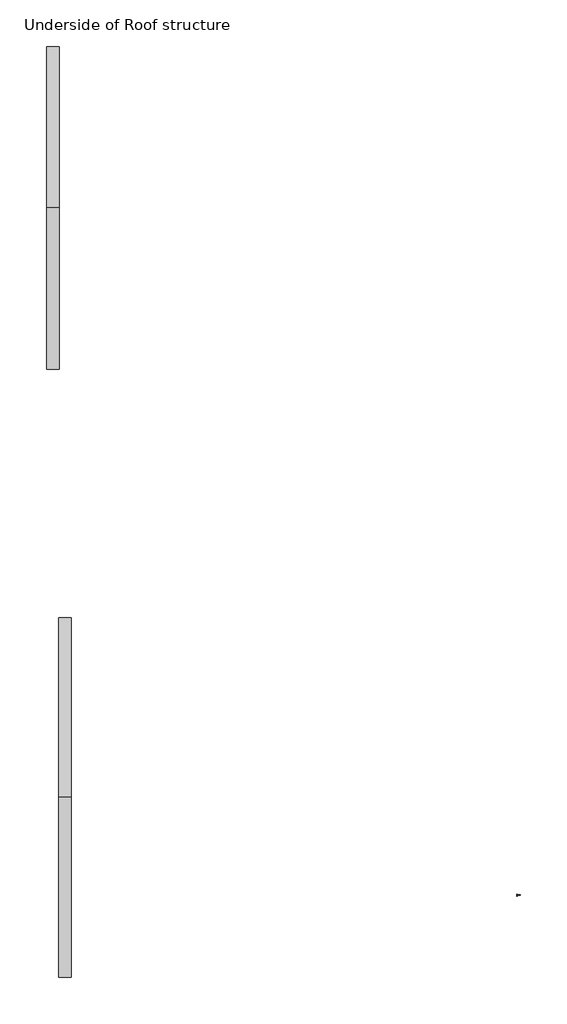
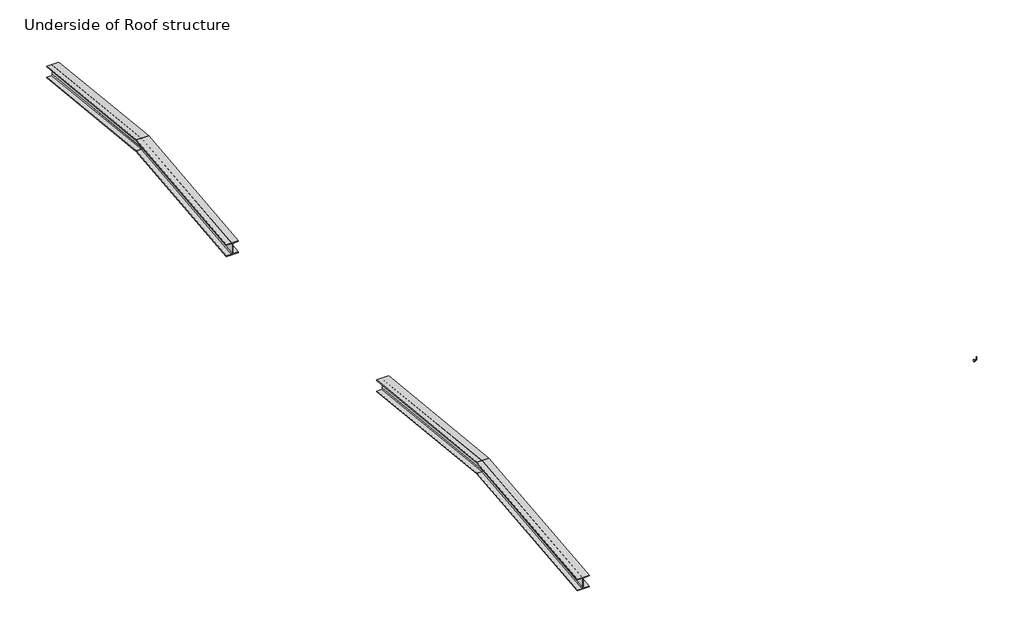
# One storey: 4 beams, 1 proxy.
"""IFC4 building model written with IfcOpenShell, lengths in millimetres."""

import ifcopenshell
import ifcopenshell.guid

model = None  # the IFC model being written
_history = None  # IfcOwnerHistory: only IFC2X3 demands one
_inside = {}  # id of a spatial element -> (the spatial element, [elements in it])
_under = {}  # id of a project, library or spatial element -> (it, [spatial elements below it])
_declared = {}  # id of a project -> (the project, [libraries it declares])
_typed = {}  # id of a type object -> (the type object, [elements of that type])
_made_of = {}  # id of a material, layer set ... -> (it, [elements and type objects made of it])


def new_model(schema):
    """Start an empty IFC model of exactly this schema.

    Asked for "IFC4X3", IfcOpenShell would pick the latest addendum, in which some entities
    have other attributes; the version numbers below select the first issue.
    IFC2X3 requires an IfcOwnerHistory on every rooted entity: one is made here for all.
    """
    global model, _history
    if schema == "IFC4X3":
        model = ifcopenshell.file(schema_version=(4, 3, 0, 0))
    else:
        model = ifcopenshell.file(schema=schema)
    _inside.clear()
    _under.clear()
    _declared.clear()
    _typed.clear()
    _made_of.clear()
    _history = None
    if model.schema == "IFC2X3":
        org = make("IfcOrganization", Name="unknown")
        user = make(
            "IfcPersonAndOrganization",
            ThePerson=make("IfcPerson", FamilyName="unknown"),
            TheOrganization=org,
        )
        app = make(
            "IfcApplication",
            ApplicationDeveloper=org,
            Version="unknown",
            ApplicationFullName="unknown",
            ApplicationIdentifier="unknown",
        )
        _history = make(
            "IfcOwnerHistory",
            OwningUser=user,
            OwningApplication=app,
            ChangeAction="ADDED",
            CreationDate=0,
        )
    return model


def make(cls, **values):
    """One entity of the class cls with the attributes given. An attribute that is None is left unset."""
    return model.create_entity(
        cls, **{name: value for name, value in values.items() if value is not None}
    )


def rooted(cls, **values):
    """An entity with a GlobalId (a new one), such as an element, a storey or a relation."""
    return make(cls, GlobalId=ifcopenshell.guid.new(), OwnerHistory=_history, **values)


def si_unit(unit_type, name, prefix=None):
    """IfcSIUnit, for example si_unit("LENGTHUNIT", "METRE", prefix="MILLI")."""
    return make("IfcSIUnit", UnitType=unit_type, Prefix=prefix, Name=name)


def assignment(units):
    """IfcUnitAssignment: the units of a project."""
    return None if units is None else make("IfcUnitAssignment", Units=units)


def point(xyz):
    """IfcCartesianPoint."""
    return None if xyz is None else make("IfcCartesianPoint", Coordinates=xyz)


def direction(xyz):
    """IfcDirection."""
    return None if xyz is None else make("IfcDirection", DirectionRatios=xyz)


def frame(location, z_axis=None, x_axis=None):
    """IfcAxis2Placement3D, a coordinate frame: its origin and axes. An axis left out is left unset."""
    return make(
        "IfcAxis2Placement3D",
        Location=point(location),
        Axis=direction(z_axis),
        RefDirection=direction(x_axis),
    )


def frame_2d(location, x_axis=None):
    """IfcAxis2Placement2D, a coordinate frame in the plane: its origin and x axis."""
    return make(
        "IfcAxis2Placement2D", Location=point(location), RefDirection=direction(x_axis)
    )


def origin():
    """The frame at (0, 0, 0) with its axes left unset."""
    return frame((0.0, 0.0, 0.0))


def origin_with_axes():
    """The frame at (0, 0, 0) with the z axis (0, 0, 1) and the x axis (1, 0, 0) written out."""
    return frame((0.0, 0.0, 0.0), z_axis=(0.0, 0.0, 1.0), x_axis=(1.0, 0.0, 0.0))


def place(relative_to, where):
    """IfcLocalPlacement: puts the frame where relative to a parent placement (None: the world)."""
    return make(
        "IfcLocalPlacement", PlacementRelTo=relative_to, RelativePlacement=where
    )


def context(
    kind, dimensions, precision=None, world=None, true_north=None, identifier=None
):
    """IfcGeometricRepresentationContext, for example the 3D "Model" context."""
    return make(
        "IfcGeometricRepresentationContext",
        ContextIdentifier=identifier,
        ContextType=kind,
        CoordinateSpaceDimension=dimensions,
        Precision=precision,
        WorldCoordinateSystem=world,
        TrueNorth=true_north,
    )


def project(units=None, contexts=None):
    """IfcProject with its units and contexts."""
    return rooted(
        "IfcProject",
        Name="project",
        RepresentationContexts=contexts,
        UnitsInContext=assignment(units),
    )


def spatial(cls, under=None, at=None, **own):
    """A site, building, storey or space (cls), placed at a placement, below another one or the project."""
    s = rooted(cls, ObjectPlacement=at, **own)
    if under is not None:
        _under.setdefault(under.id(), (under, []))[1].append(s)
    return s


def polyline(points):
    """IfcPolyline through the points."""
    return make("IfcPolyline", Points=[point(p) for p in points])


def circle_curve(where, radius):
    """IfcCircle in the frame where."""
    return make("IfcCircle", Position=where, Radius=radius)


def ellipse_curve(where, semi_axis1, semi_axis2):
    """IfcEllipse in the frame where."""
    return make(
        "IfcEllipse", Position=where, SemiAxis1=semi_axis1, SemiAxis2=semi_axis2
    )


def trimmed(basis, trim1, trim2, sense, master):
    """IfcTrimmedCurve: the piece of a basis curve between two trims."""
    return make(
        "IfcTrimmedCurve",
        BasisCurve=basis,
        Trim1=trim1,
        Trim2=trim2,
        SenseAgreement=sense,
        MasterRepresentation=master,
    )


def segment(curve, same_sense, transition):
    """IfcCompositeCurveSegment."""
    return make(
        "IfcCompositeCurveSegment",
        Transition=transition,
        SameSense=same_sense,
        ParentCurve=curve,
    )


def composite_curve(segments, self_intersect=None):
    """IfcCompositeCurve: segments joined end to end."""
    return make("IfcCompositeCurve", Segments=segments, SelfIntersect=self_intersect)


def outline(outer, holes=None, kind="AREA"):
    """IfcArbitraryClosedProfileDef: a profile drawn as a closed curve; with holes, ...WithVoids."""
    if holes is None:
        return make("IfcArbitraryClosedProfileDef", ProfileType=kind, OuterCurve=outer)
    return make(
        "IfcArbitraryProfileDefWithVoids",
        ProfileType=kind,
        OuterCurve=outer,
        InnerCurves=holes,
    )


def extrude(swept, where, along, depth):
    """IfcExtrudedAreaSolid: the profile swept, set in the frame where, extruded along a direction by depth."""
    return make(
        "IfcExtrudedAreaSolid",
        SweptArea=swept,
        Position=where,
        ExtrudedDirection=direction(along),
        Depth=depth,
    )


def shape(context_of_items, identifier, shape_type, items):
    """IfcShapeRepresentation: the items that make up one representation, for example the "Body"."""
    return make(
        "IfcShapeRepresentation",
        ContextOfItems=context_of_items,
        RepresentationIdentifier=identifier,
        RepresentationType=shape_type,
        Items=items,
    )


def source(mapping_origin, context_of_items, identifier, shape_type, items):
    """IfcRepresentationMap: a shape defined once, which mapped items show again and again."""
    return make(
        "IfcRepresentationMap",
        MappingOrigin=mapping_origin,
        MappedRepresentation=shape(context_of_items, identifier, shape_type, items),
    )


def transform(
    local_origin,
    x_axis=None,
    y_axis=None,
    z_axis=None,
    scale=None,
    scale2=None,
    scale3=None,
    uniform=True,
):
    """IfcCartesianTransformationOperator3D, or its non-uniform kind. x_axis, y_axis, z_axis: its Axis1, 2, 3."""
    if uniform:
        return make(
            "IfcCartesianTransformationOperator3D",
            Axis1=direction(x_axis),
            Axis2=direction(y_axis),
            LocalOrigin=point(local_origin),
            Scale=scale,
            Axis3=direction(z_axis),
        )
    return make(
        "IfcCartesianTransformationOperator3DnonUniform",
        Axis1=direction(x_axis),
        Axis2=direction(y_axis),
        LocalOrigin=point(local_origin),
        Scale=scale,
        Axis3=direction(z_axis),
        Scale2=scale2,
        Scale3=scale3,
    )


def mapped(mapping_source, mapping_target):
    """IfcMappedItem: shows the shape of a source again, moved by a transform."""
    return make(
        "IfcMappedItem", MappingSource=mapping_source, MappingTarget=mapping_target
    )


def made_of(thing, what):
    """Note that an element or type object is made of a material, layer set ...; save() writes the relation."""
    if what is not None:
        _made_of.setdefault(what.id(), (what, []))[1].append(thing)
    return thing


def element(
    cls,
    number,
    at=None,
    inside=None,
    cuts=None,
    type_object=None,
    material=None,
    context=None,
    identifier="Body",
    shape_type=None,
    held_by="IfcProductDefinitionShape",
    body=None,
    shapes=None,
    **own,
):
    """One element of the class cls, such as IfcWall. Its Tag is "e" and its number.

    at: its placement. inside: the storey or other place that contains it. cuts: it is an
    opening in that element (IfcRelVoidsElement). A single representation is given by context,
    identifier, shape_type and body (its items); several are given by shapes. held_by: the class
    of the entity that holds the representations. save() writes the other relations.
    """
    e = rooted(cls, Tag="e%d" % number, ObjectPlacement=at, **own)
    if body is not None:
        shapes = [shape(context, identifier, shape_type, body)]
    if shapes is not None:
        e.Representation = make(held_by, Representations=shapes)
    if inside is not None:
        _inside.setdefault(inside.id(), (inside, []))[1].append(e)
    if cuts is not None:
        rooted(
            "IfcRelVoidsElement", RelatingBuildingElement=cuts, RelatedOpeningElement=e
        )
    if type_object is not None:
        _typed.setdefault(type_object.id(), (type_object, []))[1].append(e)
    return made_of(e, material)


def aggregate(whole, parts):
    """IfcRelAggregates: a whole, such as a stair, and the parts it consists of."""
    return rooted("IfcRelAggregates", RelatingObject=whole, RelatedObjects=parts)


def save(model, path):
    """Write the relations noted so far, then the file.

    IfcRelAggregates (storeys below a building ...), IfcRelContainedInSpatialStructure (elements
    in a storey), IfcRelDefinesByType, IfcRelAssociatesMaterial and IfcRelDeclares: one each for
    every whole, place, type object, material and project.
    """
    for whole, parts in _under.values():
        aggregate(whole, parts)
    for where, things in _inside.values():
        rooted(
            "IfcRelContainedInSpatialStructure",
            RelatedElements=things,
            RelatingStructure=where,
        )
    for kind, things in _typed.values():
        rooted("IfcRelDefinesByType", RelatedObjects=things, RelatingType=kind)
    for what, things in _made_of.values():
        rooted("IfcRelAssociatesMaterial", RelatedObjects=things, RelatingMaterial=what)
    for by, libraries in _declared.values():
        rooted("IfcRelDeclares", RelatingContext=by, RelatedDefinitions=libraries)
    model.write(path)


def plane_surface(at):
    """IfcPlane: the flat surface through the origin of the frame at, square to its z axis."""
    return make("IfcPlane", Position=at)


def cylinder_surface(at, radius):
    """IfcCylindricalSurface: all points at the distance radius from the z axis of the frame at."""
    return make("IfcCylindricalSurface", Position=at, Radius=radius)


def revolved_surface(curve, axis_point, axis_direction):
    """IfcSurfaceOfRevolution: the curve turned about the line through axis_point along axis_direction."""
    return make(
        "IfcSurfaceOfRevolution",
        SweptCurve=make("IfcArbitraryOpenProfileDef", ProfileType="CURVE", Curve=curve),
        AxisPosition=make("IfcAxis1Placement", Location=point(axis_point), Axis=direction(axis_direction)),
    )


def advanced_brep(points, edges, surfaces, faces):
    """IfcAdvancedBrep: a solid bounded by faces that lie on surfaces and meet in shared edges.

    An edge is (start, end): straight between two places in points (the first is 0);
    or (start, end, curve); or (start, end, curve, False) where it runs against its curve.
    A face is (place in surfaces, loops), or (place, loops, False) where it looks against
    its surface's normal. A loop lists edges by number (the first is 1), with a minus sign
    where the edge is run from its end to its start. The first loop is the outer one.
    """
    corners = [point(p) for p in points]
    vertices = [make("IfcVertexPoint", VertexGeometry=c) for c in corners]
    made = []
    for start, end, *more in edges:
        made.append(
            make(
                "IfcEdgeCurve",
                EdgeStart=vertices[start],
                EdgeEnd=vertices[end],
                EdgeGeometry=more[0] if more else make("IfcPolyline", Points=[corners[start], corners[end]]),
                SameSense=more[1] if len(more) > 1 else True,
            )
        )
    hull = []
    for where, loops, *sense in faces:
        bounds = []
        for j, loop in enumerate(loops):
            ring = [make("IfcOrientedEdge", EdgeElement=made[abs(k) - 1], Orientation=k > 0) for k in loop]
            bounds.append(
                make(
                    "IfcFaceOuterBound" if j == 0 else "IfcFaceBound",
                    Bound=make("IfcEdgeLoop", EdgeList=ring),
                    Orientation=True,
                )
            )
        hull.append(make("IfcAdvancedFace", Bounds=bounds, FaceSurface=surfaces[where], SameSense=sense[0] if sense else True))
    return make("IfcAdvancedBrep", Outer=make("IfcClosedShell", CfsFaces=hull))


def support_metal_circular1_support_metal_circular_6fb01533(model_context):
    return source(origin(), model_context, "Body", "SolidModel", [
        advanced_brep(
        [(0.0, 63.5, -69.85), (0.0, 63.5, -82.55), (0.0, 12.7, -69.85), (0.0, 12.7, -82.55), (0.0, -6.35, -63.5), (0.0, 6.35, -63.5), (0.0, 6.35, 0.0), (0.0, -6.35, 0.0)],
        [
            (0, 1, circle_curve(frame((0.0, 63.5, -76.2), z_axis=(0.0, 1.0, 0.0), x_axis=(0.0, 0.0, -1.0)), 6.35)),
            (1, 0, circle_curve(frame((0.0, 63.5, -76.2), z_axis=(0.0, 1.0, 0.0), x_axis=(0.0, 0.0, -1.0)), 6.35)),
            (0, 2),
            (2, 3, circle_curve(frame((0.0, 12.7, -76.2), z_axis=(0.0, 1.0, 0.0), x_axis=(0.0, 0.0, -1.0)), 6.35)),
            (3, 1),
            (3, 2, circle_curve(frame((0.0, 12.7, -76.2), z_axis=(0.0, 1.0, 0.0), x_axis=(0.0, 0.0, -1.0)), 6.35)),
            (4, 3, circle_curve(frame((0.0, 12.7, -63.5), z_axis=(1.0, 0.0, 0.0), x_axis=(0.0, 0.0, -1.0)), 19.05)),
            (2, 5, circle_curve(frame((0.0, 12.7, -63.5), z_axis=(-1.0, 0.0, 0.0), x_axis=(0.0, 0.0, -1.0)), 6.35)),
            (5, 4, circle_curve(frame((0.0, 0.0, -63.5), z_axis=(0.0, 0.0, -1.0), x_axis=(0.0, -1.0, 0.0)), 6.35)),
            (4, 5, circle_curve(frame((0.0, 0.0, -63.5), z_axis=(0.0, 0.0, -1.0), x_axis=(0.0, -1.0, 0.0)), 6.35)),
            (6, 7, circle_curve(frame((0.0, 0.0, 0.0), z_axis=(0.0, 0.0, 1.0), x_axis=(0.0, -1.0, 0.0)), 6.35)),
            (7, 6, circle_curve(frame((0.0, 0.0, 0.0), z_axis=(0.0, 0.0, 1.0), x_axis=(0.0, -1.0, 0.0)), 6.35)),
            (5, 6),
            (7, 4),
        ],
        [
            plane_surface(frame((0.0, 63.5, -76.2), z_axis=(0.0, 1.0, 0.0), x_axis=(1.0, 0.0, 0.0))),
            cylinder_surface(frame((0.0, 63.5, -76.2), z_axis=(0.0, 1.0, 0.0), x_axis=(0.0, 0.0, -1.0)), 6.35),
            revolved_surface(trimmed(ellipse_curve(frame((0.0, 12.7, -76.2), z_axis=(0.0, 1.0, 0.0), x_axis=(0.0, 0.0, -1.0)), 6.35, 6.35), [point((0.0, 12.7, -69.85))], [point((0.0, 12.7, -82.55))], True, "CARTESIAN"), (0.0, 12.7, -63.5), (-1.0, 0.0, 0.0)),
            revolved_surface(trimmed(ellipse_curve(frame((0.0, 12.7, -76.2), z_axis=(0.0, 1.0, 0.0), x_axis=(0.0, 0.0, -1.0)), 6.35, 6.35), [point((0.0, 12.7, -82.55))], [point((0.0, 12.7, -69.85))], True, "CARTESIAN"), (0.0, 12.7, -63.5), (-1.0, 0.0, 0.0)),
            plane_surface(origin_with_axes()),
            cylinder_surface(frame((0.0, 0.0, -63.5), z_axis=(0.0, 0.0, -1.0), x_axis=(0.0, -1.0, 0.0)), 6.35),
        ],
        [
            (0, [[1, 2]]),
            (1, [[-1, 3, 4, 5]]),
            (1, [[-2, -5, 6, -3]]),
            (2, [[7, -4, 8, 9]]),
            (3, [[-8, -6, -7, 10]]),
            (4, [[11, 12]]),
            (5, [[-9, 13, -12, 14]]),
            (5, [[-10, -14, -11, -13]]),
        ],
    ),
        extrude(outline(composite_curve([segment(trimmed(circle_curve(frame_2d((-76.2, 0.0)), 25.4), [point((-76.2, -25.4))], [point((-76.2, 25.4))], False, "CARTESIAN"), True, "CONTINUOUS"), segment(trimmed(circle_curve(frame_2d((-76.2, 0.0)), 25.4), [point((-76.2, 25.4))], [point((-76.2, -25.4))], False, "CARTESIAN"), True, "CONTINUOUS")], self_intersect=False)), frame((0.0, 63.5, 0.0), z_axis=(0.0, 1.0, 0.0), x_axis=(0.0, 0.0, 1.0)), (0.0, 0.0, 1.0), 12.7),
    ])


model = new_model("IFC4")

# Units and contexts
model_context = context("Model", 3, world=origin())
ifc_project = project(units=[si_unit("LENGTHUNIT", "METRE", prefix="MILLI")], contexts=[model_context])

# Site, building, storey
site = spatial("IfcSite", under=ifc_project)
building = spatial("IfcBuilding", under=site)
storey = spatial("IfcBuildingStorey", under=building, Name="Underside of Roof structure", Elevation=34036.0)

# Beams
placement = place(None, origin())
element("IfcBeam", 1, ObjectType="W-Wide Flange : W12X79", at=placement, inside=storey, context=model_context, shape_type="AdvancedBrep", body=[
    advanced_brep(
    [(-21755.4154607, 20844.8695005, 33191.9562864), (-21755.4154607, 16882.4695005, 33611.0562864), (-21630.3204607, 16882.4695005, 33611.0562864), (-21630.3204607, 20844.8695005, 33191.9562864), (-21755.4154607, 20844.8695005, 33173.1831506), (-21755.4154607, 16882.4695005, 33592.2831506), (-21448.0754607, 16882.4695005, 33592.2831506), (-21448.0754607, 16882.4695005, 33611.0562864), (-21573.1704607, 16882.4695005, 33611.0562864), (-21595.7764607, 16882.4695005, 33633.7883829), (-21595.7764607, 16882.4695005, 33867.4947677), (-21573.1704607, 16882.4695005, 33890.2268642), (-21448.0754607, 16882.4695005, 33890.2268642), (-21448.0754607, 16882.4695005, 33909.0), (-21755.4154607, 16882.4695005, 33909.0), (-21755.4154607, 16882.4695005, 33890.2268642), (-21630.3204607, 16882.4695005, 33890.2268642), (-21607.7144607, 16882.4695005, 33867.4947677), (-21607.7144607, 16882.4695005, 33633.7883829), (-21607.7144607, 20844.8695005, 33214.6883829), (-21607.7144607, 20844.8695005, 33448.3947677), (-21630.3204607, 20844.8695005, 33471.1268642), (-21755.4154607, 20844.8695005, 33471.1268642), (-21755.4154607, 20844.8695005, 33489.9), (-21448.0754607, 20844.8695005, 33489.9), (-21448.0754607, 20844.8695005, 33471.1268642), (-21573.1704607, 20844.8695005, 33471.1268642), (-21595.7764607, 20844.8695005, 33448.3947677), (-21595.7764607, 20844.8695005, 33214.6883829), (-21573.1704607, 20844.8695005, 33191.9562864), (-21448.0754607, 20844.8695005, 33191.9562864), (-21448.0754607, 20844.8695005, 33173.1831506)],
    [
        (0, 1),
        (1, 2),
        (2, 3),
        (3, 0),
        (4, 5),
        (5, 1),
        (0, 4),
        (5, 6),
        (6, 7),
        (7, 8),
        (8, 9, ellipse_curve(frame((-21573.1704607, 16882.4695005, 33633.7883829), z_axis=(0.0, 1.0, 0.0), x_axis=(0.0, 0.0, 0.9999999999999999)), 22.7320964, 22.606)),
        (9, 10),
        (10, 11, ellipse_curve(frame((-21573.1704607, 16882.4695005, 33867.4947677), z_axis=(0.0, 1.0, 0.0), x_axis=(0.0, 0.0, 0.9999999999999999)), 22.7320964, 22.606)),
        (11, 12),
        (12, 13),
        (13, 14),
        (14, 15),
        (15, 16),
        (16, 17, ellipse_curve(frame((-21630.3204607, 16882.4695005, 33867.4947677), z_axis=(0.0, 1.0, 0.0), x_axis=(0.0, 0.0, 0.9999999999999999)), 22.7320964, 22.606)),
        (17, 18),
        (18, 2, ellipse_curve(frame((-21630.3204607, 16882.4695005, 33633.7883829), z_axis=(0.0, 1.0, 0.0), x_axis=(0.0, 0.0, 0.9999999999999999)), 22.7320964, 22.606)),
        (18, 19),
        (19, 3, ellipse_curve(frame((-21630.3204607, 20844.8695005, 33214.6883829), z_axis=(0.0, 1.0, 0.0), x_axis=(0.0, 0.0, 0.9999999999999999)), 22.7320964, 22.606)),
        (17, 20),
        (20, 19),
        (16, 21),
        (21, 20, ellipse_curve(frame((-21630.3204607, 20844.8695005, 33448.3947677), z_axis=(0.0, 1.0, 0.0), x_axis=(0.0, 0.0, 0.9999999999999999)), 22.7320964, 22.606)),
        (15, 22),
        (22, 21),
        (14, 23),
        (23, 22),
        (13, 24),
        (24, 23),
        (12, 25),
        (25, 24),
        (11, 26),
        (26, 25),
        (10, 27),
        (27, 26, ellipse_curve(frame((-21573.1704607, 20844.8695005, 33448.3947677), z_axis=(0.0, 1.0, 0.0), x_axis=(0.0, 0.0, 0.9999999999999999)), 22.7320964, 22.606)),
        (9, 28),
        (28, 27),
        (8, 29),
        (29, 28, ellipse_curve(frame((-21573.1704607, 20844.8695005, 33214.6883829), z_axis=(0.0, 1.0, 0.0), x_axis=(0.0, 0.0, 0.9999999999999999)), 22.7320964, 22.606)),
        (7, 30),
        (30, 29),
        (6, 31),
        (31, 30),
        (4, 31),
    ],
    [
        plane_surface(frame((-21692.8679607, 20969.2190095, 33178.8039345), z_axis=(0.0, 0.10518252182083103, 0.9944529335787644), x_axis=(1.0, 0.0, 0.0))),
        plane_surface(frame((-21755.4154607, 20968.2371832, 33169.5212136), z_axis=(-1.0, 0.0, 0.0), x_axis=(0.0, 0.10518252182083183, 0.9944529335787644))),
        plane_surface(frame((-21601.7454607, 16882.4695005, 33592.2831506), z_axis=(0.0, -1.0, 0.0), x_axis=(0.0, 0.0, 1.0))),
        revolved_surface(polyline([(-21607.7144607, 16880.091744411304, 33634.03987627958), (-21607.7144607, 20847.247256588096, 33214.43688941473)]), (-21630.3204607, 20971.5967656, 33201.2845375), (0.0, -0.9944529335787643, 0.10518252182083102)),
        plane_surface(frame((-21607.7144607, 20983.8195005, 33316.8449407), z_axis=(-1.0, 0.0, 0.0), x_axis=(0.0, 0.10518252182083183, 0.9944529335787644))),
        revolved_surface(polyline([(-21630.3204607, 16882.46950049405, 33890.226864143755), (-21630.3204607, 20849.625012670844, 33470.6238772789)]), (-21630.3204607, 20996.0422355, 33432.4053438), (0.0, -0.9944529335787643, 0.10518252182083102)),
        plane_surface(frame((-21692.8679607, 20998.4199915, 33454.8859468), z_axis=(0.0, -0.10518252182083103, -0.9944529335787644), x_axis=(-1.0, 0.0, 0.0))),
        plane_surface(frame((-21755.4154607, 20999.4018178, 33464.1686678), z_axis=(-1.0, 0.0, 0.0), x_axis=(0.0, 0.10518252182083183, 0.9944529335787644))),
        plane_surface(frame((-21601.7454607, 21000.383644, 33473.4513887), z_axis=(0.0, 0.10518252182083103, 0.9944529335787644), x_axis=(1.0, 0.0, 0.0))),
        plane_surface(frame((-21448.0754607, 20999.4018178, 33464.1686678), z_axis=(1.0, 0.0, 0.0), x_axis=(0.0, -0.10518252182083183, -0.9944529335787644))),
        plane_surface(frame((-21510.6229607, 20998.4199915, 33454.8859468), z_axis=(0.0, -0.10518252182083103, -0.9944529335787644), x_axis=(-1.0, 0.0, 0.0))),
        revolved_surface(polyline([(-21595.7764607, 16880.09174440577, 33867.74626112727), (-21595.7764607, 20847.247256582563, 33448.14327426242)]), (-21573.1704607, 20996.0422355, 33432.4053438), (0.0, -0.9944529335787643, 0.10518252182083102)),
        plane_surface(frame((-21595.7764607, 20983.8195005, 33316.8449407), z_axis=(1.0, 0.0, 0.0), x_axis=(0.0, -0.10518252182083183, -0.9944529335787644))),
        revolved_surface(polyline([(-21573.1704607, 16877.713988323023, 33611.5592732631), (-21573.1704607, 20844.869500499815, 33191.95628639824)]), (-21573.1704607, 20971.5967656, 33201.2845375), (0.0, -0.9944529335787643, 0.10518252182083102)),
        plane_surface(frame((-21510.6229607, 20969.2190095, 33178.8039345), z_axis=(0.0, 0.10518252182083103, 0.9944529335787644), x_axis=(1.0, 0.0, 0.0))),
        plane_surface(frame((-21448.0754607, 20968.2371832, 33169.5212136), z_axis=(1.0, 0.0, 0.0), x_axis=(0.0, -0.10518252182083183, -0.9944529335787644))),
        plane_surface(frame((-21601.7454607, 20967.255357, 33160.2384927), z_axis=(0.0, -0.10518252182083103, -0.9944529335787644), x_axis=(-1.0, 0.0, 0.0))),
        plane_surface(frame((-23272.9998994, 20844.8695005, 33801.3683204), z_axis=(0.0, 1.0, 0.0), x_axis=(0.0, 0.0, 1.0))),
    ],
    [
        (0, [[1, 2, 3, 4]]),
        (1, [[5, 6, -1, 7]]),
        (2, [[-6, 8, 9, 10, 11, 12, 13, 14, 15, 16, 17, 18, 19, 20, 21, -2]]),
        (3, [[-3, -21, 22, 23]]),
        (4, [[-22, -20, 24, 25]]),
        (5, [[-24, -19, 26, 27]]),
        (6, [[-26, -18, 28, 29]]),
        (7, [[-28, -17, 30, 31]]),
        (8, [[-30, -16, 32, 33]]),
        (9, [[-32, -15, 34, 35]]),
        (10, [[-34, -14, 36, 37]]),
        (11, [[-36, -13, 38, 39]]),
        (12, [[-38, -12, 40, 41]]),
        (13, [[-40, -11, 42, 43]]),
        (14, [[-42, -10, 44, 45]]),
        (15, [[-44, -9, 46, 47]]),
        (16, [[-46, -8, -5, 48]]),
        (17, [[-4, -23, -25, -27, -29, -31, -33, -35, -37, -39, -41, -43, -45, -47, -48, -7]]),
    ],
),
])
element("IfcBeam", 2, ObjectType="W-Wide Flange : W12X79", at=placement, inside=storey, context=model_context, shape_type="AdvancedBrep", body=[
    advanced_brep(
    [(-21607.7144607, 12920.0695005, 33214.6883829), (-21607.7144607, 16882.4695005, 33633.7883829), (-21630.3204607, 16882.4695005, 33611.0562864), (-21630.3204607, 12920.0695005, 33191.9562864), (-21755.4154607, 16882.4695005, 33611.0562864), (-21755.4154607, 12920.0695005, 33191.9562864), (-21607.7144607, 16882.4695005, 33867.4947677), (-21630.3204607, 16882.4695005, 33890.2268642), (-21755.4154607, 16882.4695005, 33890.2268642), (-21755.4154607, 16882.4695005, 33909.0), (-21448.0754607, 16882.4695005, 33909.0), (-21448.0754607, 16882.4695005, 33890.2268642), (-21573.1704607, 16882.4695005, 33890.2268642), (-21595.7764607, 16882.4695005, 33867.4947677), (-21595.7764607, 16882.4695005, 33633.7883829), (-21573.1704607, 16882.4695005, 33611.0562864), (-21448.0754607, 16882.4695005, 33611.0562864), (-21448.0754607, 16882.4695005, 33592.2831506), (-21755.4154607, 16882.4695005, 33592.2831506), (-21755.4154607, 12920.0695005, 33173.1831506), (-21607.7144607, 12920.0695005, 33448.3947677), (-21630.3204607, 12920.0695005, 33471.1268642), (-21755.4154607, 12920.0695005, 33471.1268642), (-21755.4154607, 12920.0695005, 33489.9), (-21448.0754607, 12920.0695005, 33489.9), (-21448.0754607, 12920.0695005, 33471.1268642), (-21573.1704607, 12920.0695005, 33471.1268642), (-21595.7764607, 12920.0695005, 33448.3947677), (-21595.7764607, 12920.0695005, 33214.6883829), (-21573.1704607, 12920.0695005, 33191.9562864), (-21448.0754607, 12920.0695005, 33191.9562864), (-21448.0754607, 12920.0695005, 33173.1831506)],
    [
        (0, 1),
        (1, 2, ellipse_curve(frame((-21630.3204607, 16882.4695005, 33633.7883829), z_axis=(0.0, 1.0, 0.0), x_axis=(0.0, 0.0, 1.0)), 22.7320964, 22.606)),
        (2, 3),
        (3, 0, ellipse_curve(frame((-21630.3204607, 12920.0695005, 33214.6883829), z_axis=(0.0, -1.0, 0.0), x_axis=(0.0, 0.0, 1.0)), 22.7320964, 22.606)),
        (2, 4),
        (4, 5),
        (5, 3),
        (1, 6),
        (6, 7, ellipse_curve(frame((-21630.3204607, 16882.4695005, 33867.4947677), z_axis=(0.0, -1.0, 0.0), x_axis=(0.0, 0.0, 1.0)), 22.7320964, 22.606)),
        (7, 8),
        (8, 9),
        (9, 10),
        (10, 11),
        (11, 12),
        (12, 13, ellipse_curve(frame((-21573.1704607, 16882.4695005, 33867.4947677), z_axis=(0.0, -1.0, 0.0), x_axis=(0.0, 0.0, 1.0)), 22.7320964, 22.606)),
        (13, 14),
        (14, 15, ellipse_curve(frame((-21573.1704607, 16882.4695005, 33633.7883829), z_axis=(0.0, -1.0, 0.0), x_axis=(0.0, 0.0, 1.0)), 22.7320964, 22.606)),
        (15, 16),
        (16, 17),
        (17, 18),
        (18, 4),
        (18, 19),
        (19, 5),
        (20, 6),
        (0, 20),
        (21, 7),
        (20, 21, ellipse_curve(frame((-21630.3204607, 12920.0695005, 33448.3947677), z_axis=(0.0, -1.0, 0.0), x_axis=(0.0, 0.0, 1.0)), 22.7320964, 22.606)),
        (22, 8),
        (21, 22),
        (23, 9),
        (22, 23),
        (24, 10),
        (23, 24),
        (25, 11),
        (24, 25),
        (26, 12),
        (25, 26),
        (27, 13),
        (26, 27, ellipse_curve(frame((-21573.1704607, 12920.0695005, 33448.3947677), z_axis=(0.0, -1.0, 0.0), x_axis=(0.0, 0.0, 1.0)), 22.7320964, 22.606)),
        (28, 14),
        (27, 28),
        (29, 15),
        (28, 29, ellipse_curve(frame((-21573.1704607, 12920.0695005, 33214.6883829), z_axis=(0.0, -1.0, 0.0), x_axis=(0.0, 0.0, 1.0)), 22.7320964, 22.606)),
        (30, 16),
        (29, 30),
        (31, 17),
        (30, 31),
        (31, 19),
    ],
    [
        revolved_surface(polyline([(-21607.7144607, 16884.847256589805, 33634.03987626912), (-21607.7144607, 12917.69174441301, 33214.436889404264)]), (-21630.3204607, 12793.3422355, 33201.2845375), (0.0, 0.9944529335787644, 0.10518252182083103)),
        plane_surface(frame((-21692.8679607, 12795.7199915, 33178.8039345), z_axis=(0.0, -0.10518252182083103, 0.9944529335787644), x_axis=(1.0, 0.0, 0.0))),
        plane_surface(frame((-21601.7454607, 16882.4695005, 33592.2831506), z_axis=(0.0, 1.0, 0.0), x_axis=(0.0, 0.0, -1.0))),
        plane_surface(frame((-21755.4154607, 12796.7018178, 33169.5212136), z_axis=(-1.0, 0.0, 0.0), x_axis=(0.0, -0.10518252182083185, 0.9944529335787644))),
        plane_surface(frame((-21607.7144607, 12781.1195005, 33316.8449407), z_axis=(-1.0, 0.0, 0.0), x_axis=(0.0, -0.10518252182083185, 0.9944529335787644))),
        revolved_surface(polyline([(-21630.3204607, 16882.469500507057, 33890.2268641333), (-21630.3204607, 12915.313988330263, 33470.623877268445)]), (-21630.3204607, 12768.8967656, 33432.4053438), (0.0, 0.9944529335787644, 0.10518252182083103)),
        plane_surface(frame((-21692.8679607, 12766.5190095, 33454.8859468), z_axis=(0.0, 0.10518252182083103, -0.9944529335787644), x_axis=(-1.0, 0.0, 0.0))),
        plane_surface(frame((-21755.4154607, 12765.5371832, 33464.1686678), z_axis=(-1.0, 0.0, 0.0), x_axis=(0.0, -0.10518252182083185, 0.9944529335787644))),
        plane_surface(frame((-21601.7454607, 12764.555357, 33473.4513887), z_axis=(0.0, -0.10518252182083103, 0.9944529335787644), x_axis=(1.0, 0.0, 0.0))),
        plane_surface(frame((-21448.0754607, 12765.5371832, 33464.1686678), z_axis=(1.0, 0.0, 0.0), x_axis=(0.0, 0.10518252182083185, -0.9944529335787644))),
        plane_surface(frame((-21510.6229607, 12766.5190095, 33454.8859468), z_axis=(0.0, 0.10518252182083103, -0.9944529335787644), x_axis=(-1.0, 0.0, 0.0))),
        revolved_surface(polyline([(-21595.7764607, 16884.847256595338, 33867.746261116816), (-21595.7764607, 12917.691744418544, 33448.14327425196)]), (-21573.1704607, 12768.8967656, 33432.4053438), (0.0, 0.9944529335787644, 0.10518252182083103)),
        plane_surface(frame((-21595.7764607, 12781.1195005, 33316.8449407), z_axis=(1.0, 0.0, 0.0), x_axis=(0.0, 0.10518252182083185, -0.9944529335787644))),
        revolved_surface(polyline([(-21573.1704607, 16887.225012678085, 33611.559273252635), (-21573.1704607, 12920.069500501291, 33191.95628638778)]), (-21573.1704607, 12793.3422355, 33201.2845375), (0.0, 0.9944529335787644, 0.10518252182083103)),
        plane_surface(frame((-21510.6229607, 12795.7199915, 33178.8039345), z_axis=(0.0, -0.10518252182083103, 0.9944529335787644), x_axis=(1.0, 0.0, 0.0))),
        plane_surface(frame((-21448.0754607, 12796.7018178, 33169.5212136), z_axis=(1.0, 0.0, 0.0), x_axis=(0.0, 0.10518252182083185, -0.9944529335787644))),
        plane_surface(frame((-21601.7454607, 12797.683644, 33160.2384927), z_axis=(0.0, 0.10518252182083103, -0.9944529335787644), x_axis=(-1.0, 0.0, 0.0))),
        plane_surface(frame((-23272.9998994, 12920.0695005, 33801.3683204), z_axis=(0.0, -1.0, 0.0), x_axis=(0.0, 0.0, 1.0))),
    ],
    [
        (0, [[1, 2, 3, 4]]),
        (1, [[-3, 5, 6, 7]]),
        (2, [[-5, -2, 8, 9, 10, 11, 12, 13, 14, 15, 16, 17, 18, 19, 20, 21]]),
        (3, [[-6, -21, 22, 23]]),
        (4, [[24, -8, -1, 25]]),
        (5, [[26, -9, -24, 27]]),
        (6, [[28, -10, -26, 29]]),
        (7, [[30, -11, -28, 31]]),
        (8, [[32, -12, -30, 33]]),
        (9, [[34, -13, -32, 35]]),
        (10, [[36, -14, -34, 37]]),
        (11, [[38, -15, -36, 39]]),
        (12, [[40, -16, -38, 41]]),
        (13, [[42, -17, -40, 43]]),
        (14, [[44, -18, -42, 45]]),
        (15, [[46, -19, -44, 47]]),
        (16, [[-22, -20, -46, 48]]),
        (17, [[-7, -23, -48, -47, -45, -43, -41, -39, -37, -35, -33, -31, -29, -27, -25, -4]]),
    ],
),
])
element("IfcBeam", 3, ObjectType="W-Wide Flange : W12X79", at=placement, inside=storey, context=model_context, shape_type="AdvancedBrep", body=[
    advanced_brep(
    [(-21450.6154607, 6824.0695005, 33143.5985941), (-21450.6154607, 2404.4695005, 33611.0562864), (-21325.5204607, 2404.4695005, 33611.0562864), (-21325.5204607, 6824.0695005, 33143.5985941), (-21450.6154607, 6824.0695005, 33124.8254583), (-21450.6154607, 2404.4695005, 33592.2831506), (-21143.2754607, 2404.4695005, 33592.2831506), (-21143.2754607, 2404.4695005, 33611.0562864), (-21268.3704607, 2404.4695005, 33611.0562864), (-21290.9764607, 2404.4695005, 33633.7883829), (-21290.9764607, 2404.4695005, 33867.4947677), (-21268.3704607, 2404.4695005, 33890.2268642), (-21143.2754607, 2404.4695005, 33890.2268642), (-21143.2754607, 2404.4695005, 33909.0), (-21450.6154607, 2404.4695005, 33909.0), (-21450.6154607, 2404.4695005, 33890.2268642), (-21325.5204607, 2404.4695005, 33890.2268642), (-21302.9144607, 2404.4695005, 33867.4947677), (-21302.9144607, 2404.4695005, 33633.7883829), (-21302.9144607, 6824.0695005, 33166.3306906), (-21302.9144607, 6824.0695005, 33400.0370754), (-21325.5204607, 6824.0695005, 33422.7691719), (-21450.6154607, 6824.0695005, 33422.7691719), (-21450.6154607, 6824.0695005, 33441.5423077), (-21143.2754607, 6824.0695005, 33441.5423077), (-21143.2754607, 6824.0695005, 33422.7691719), (-21268.3704607, 6824.0695005, 33422.7691719), (-21290.9764607, 6824.0695005, 33400.0370754), (-21290.9764607, 6824.0695005, 33166.3306906), (-21268.3704607, 6824.0695005, 33143.5985941), (-21143.2754607, 6824.0695005, 33143.5985941), (-21143.2754607, 6824.0695005, 33124.8254583)],
    [
        (0, 1),
        (1, 2),
        (2, 3),
        (3, 0),
        (4, 5),
        (5, 1),
        (0, 4),
        (5, 6),
        (6, 7),
        (7, 8),
        (8, 9, ellipse_curve(frame((-21268.3704607, 2404.4695005, 33633.7883829), z_axis=(0.0, 1.0, 0.0), x_axis=(0.0, 0.0, 0.9999999999999999)), 22.7320964, 22.606)),
        (9, 10),
        (10, 11, ellipse_curve(frame((-21268.3704607, 2404.4695005, 33867.4947677), z_axis=(0.0, 1.0, 0.0), x_axis=(0.0, 0.0, 0.9999999999999999)), 22.7320964, 22.606)),
        (11, 12),
        (12, 13),
        (13, 14),
        (14, 15),
        (15, 16),
        (16, 17, ellipse_curve(frame((-21325.5204607, 2404.4695005, 33867.4947677), z_axis=(0.0, 1.0, 0.0), x_axis=(0.0, 0.0, 0.9999999999999999)), 22.7320964, 22.606)),
        (17, 18),
        (18, 2, ellipse_curve(frame((-21325.5204607, 2404.4695005, 33633.7883829), z_axis=(0.0, 1.0, 0.0), x_axis=(0.0, 0.0, 0.9999999999999999)), 22.7320964, 22.606)),
        (18, 19),
        (19, 3, ellipse_curve(frame((-21325.5204607, 6824.0695005, 33166.3306906), z_axis=(0.0, 1.0, 0.0), x_axis=(0.0, 0.0, 0.9999999999999999)), 22.7320964, 22.606)),
        (17, 20),
        (20, 19),
        (16, 21),
        (21, 20, ellipse_curve(frame((-21325.5204607, 6824.0695005, 33400.0370754), z_axis=(0.0, 1.0, 0.0), x_axis=(0.0, 0.0, 0.9999999999999999)), 22.7320964, 22.606)),
        (15, 22),
        (22, 21),
        (14, 23),
        (23, 22),
        (13, 24),
        (24, 23),
        (12, 25),
        (25, 24),
        (11, 26),
        (26, 25),
        (10, 27),
        (27, 26, ellipse_curve(frame((-21268.3704607, 6824.0695005, 33400.0370754), z_axis=(0.0, 1.0, 0.0), x_axis=(0.0, 0.0, 0.9999999999999999)), 22.7320964, 22.606)),
        (9, 28),
        (28, 27),
        (8, 29),
        (29, 28, ellipse_curve(frame((-21268.3704607, 6824.0695005, 33166.3306906), z_axis=(0.0, 1.0, 0.0), x_axis=(0.0, 0.0, 0.9999999999999999)), 22.7320964, 22.606)),
        (7, 30),
        (30, 29),
        (6, 31),
        (31, 30),
        (4, 31),
    ],
    [
        plane_surface(frame((-21388.0679607, 6948.4190095, 33130.4462422), z_axis=(0.0, 0.10518252182083103, 0.9944529335787644), x_axis=(1.0, 0.0, 0.0))),
        plane_surface(frame((-21450.6154607, 6947.4371832, 33121.1635213), z_axis=(-1.0, 0.0, 0.0), x_axis=(0.0, 0.10518252182083125, 0.9944529335787644))),
        plane_surface(frame((-21296.9454607, 2404.4695005, 33592.2831506), z_axis=(0.0, -1.0, 0.0), x_axis=(0.0, 0.0, 1.0))),
        revolved_surface(polyline([(-21302.9144607, 2402.091744412107, 33634.039876287185), (-21302.9144607, 6826.447256588095, 33166.07919711473)]), (-21325.5204607, 6950.7967656, 33152.9268452), (0.0, -0.9944529335787643, 0.10518252182083102)),
        plane_surface(frame((-21302.9144607, 6963.0195005, 33268.4872484), z_axis=(-1.0, 0.0, 0.0), x_axis=(0.0, 0.10518252182083125, 0.9944529335787644))),
        revolved_surface(polyline([(-21325.5204607, 2404.4695004948553, 33890.226864151366), (-21325.5204607, 6828.825012670844, 33422.2661849789)]), (-21325.5204607, 6975.2422355, 33384.0476515), (0.0, -0.9944529335787643, 0.10518252182083102)),
        plane_surface(frame((-21388.0679607, 6977.6199915, 33406.5282545), z_axis=(0.0, -0.10518252182083103, -0.9944529335787644), x_axis=(-1.0, 0.0, 0.0))),
        plane_surface(frame((-21450.6154607, 6978.6018178, 33415.8109754), z_axis=(-1.0, 0.0, 0.0), x_axis=(0.0, 0.10518252182083125, 0.9944529335787644))),
        plane_surface(frame((-21296.9454607, 6979.583644, 33425.0936964), z_axis=(0.0, 0.10518252182083103, 0.9944529335787644), x_axis=(1.0, 0.0, 0.0))),
        plane_surface(frame((-21143.2754607, 6978.6018178, 33415.8109754), z_axis=(1.0, 0.0, 0.0), x_axis=(0.0, -0.10518252182083125, -0.9944529335787644))),
        plane_surface(frame((-21205.8229607, 6977.6199915, 33406.5282545), z_axis=(0.0, -0.10518252182083103, -0.9944529335787644), x_axis=(-1.0, 0.0, 0.0))),
        revolved_surface(polyline([(-21290.9764607, 2402.0917444065735, 33867.74626113488), (-21290.9764607, 6826.447256582563, 33399.78558196242)]), (-21268.3704607, 6975.2422355, 33384.0476515), (0.0, -0.9944529335787643, 0.10518252182083102)),
        plane_surface(frame((-21290.9764607, 6963.0195005, 33268.4872484), z_axis=(1.0, 0.0, 0.0), x_axis=(0.0, -0.10518252182083125, -0.9944529335787644))),
        revolved_surface(polyline([(-21268.3704607, 2399.713988323825, 33611.5592732707), (-21268.3704607, 6824.069500499813, 33143.59859409824)]), (-21268.3704607, 6950.7967656, 33152.9268452), (0.0, -0.9944529335787643, 0.10518252182083102)),
        plane_surface(frame((-21205.8229607, 6948.4190095, 33130.4462422), z_axis=(0.0, 0.10518252182083103, 0.9944529335787644), x_axis=(1.0, 0.0, 0.0))),
        plane_surface(frame((-21143.2754607, 6947.4371832, 33121.1635213), z_axis=(1.0, 0.0, 0.0), x_axis=(0.0, -0.10518252182083125, -0.9944529335787644))),
        plane_surface(frame((-21296.9454607, 6946.455357, 33111.8808004), z_axis=(0.0, -0.10518252182083103, -0.9944529335787644), x_axis=(-1.0, 0.0, 0.0))),
        plane_surface(frame((-23272.9998994, 6824.0695005, 33801.3683204), z_axis=(0.0, 1.0, 0.0), x_axis=(0.0, 0.0, 1.0))),
    ],
    [
        (0, [[1, 2, 3, 4]]),
        (1, [[5, 6, -1, 7]]),
        (2, [[-6, 8, 9, 10, 11, 12, 13, 14, 15, 16, 17, 18, 19, 20, 21, -2]]),
        (3, [[-3, -21, 22, 23]]),
        (4, [[-22, -20, 24, 25]]),
        (5, [[-24, -19, 26, 27]]),
        (6, [[-26, -18, 28, 29]]),
        (7, [[-28, -17, 30, 31]]),
        (8, [[-30, -16, 32, 33]]),
        (9, [[-32, -15, 34, 35]]),
        (10, [[-34, -14, 36, 37]]),
        (11, [[-36, -13, 38, 39]]),
        (12, [[-38, -12, 40, 41]]),
        (13, [[-40, -11, 42, 43]]),
        (14, [[-42, -10, 44, 45]]),
        (15, [[-44, -9, 46, 47]]),
        (16, [[-46, -8, -5, 48]]),
        (17, [[-4, -23, -25, -27, -29, -31, -33, -35, -37, -39, -41, -43, -45, -47, -48, -7]]),
    ],
),
])
element("IfcBeam", 4, ObjectType="W-Wide Flange : W12X79", at=placement, inside=storey, context=model_context, shape_type="AdvancedBrep", body=[
    advanced_brep(
    [(-21302.9144607, -2015.1304995, 33166.3306906), (-21302.9144607, 2404.4695005, 33633.7883829), (-21325.5204607, 2404.4695005, 33611.0562864), (-21325.5204607, -2015.1304995, 33143.5985941), (-21450.6154607, 2404.4695005, 33611.0562864), (-21450.6154607, -2015.1304995, 33143.5985941), (-21302.9144607, 2404.4695005, 33867.4947677), (-21325.5204607, 2404.4695005, 33890.2268642), (-21450.6154607, 2404.4695005, 33890.2268642), (-21450.6154607, 2404.4695005, 33909.0), (-21143.2754607, 2404.4695005, 33909.0), (-21143.2754607, 2404.4695005, 33890.2268642), (-21268.3704607, 2404.4695005, 33890.2268642), (-21290.9764607, 2404.4695005, 33867.4947677), (-21290.9764607, 2404.4695005, 33633.7883829), (-21268.3704607, 2404.4695005, 33611.0562864), (-21143.2754607, 2404.4695005, 33611.0562864), (-21143.2754607, 2404.4695005, 33592.2831506), (-21450.6154607, 2404.4695005, 33592.2831506), (-21450.6154607, -2015.1304995, 33124.8254583), (-21302.9144607, -2015.1304995, 33400.0370754), (-21325.5204607, -2015.1304995, 33422.7691719), (-21450.6154607, -2015.1304995, 33422.7691719), (-21450.6154607, -2015.1304995, 33441.5423077), (-21143.2754607, -2015.1304995, 33441.5423077), (-21143.2754607, -2015.1304995, 33422.7691719), (-21268.3704607, -2015.1304995, 33422.7691719), (-21290.9764607, -2015.1304995, 33400.0370754), (-21290.9764607, -2015.1304995, 33166.3306906), (-21268.3704607, -2015.1304995, 33143.5985941), (-21143.2754607, -2015.1304995, 33143.5985941), (-21143.2754607, -2015.1304995, 33124.8254583)],
    [
        (0, 1),
        (1, 2, ellipse_curve(frame((-21325.5204607, 2404.4695005, 33633.7883829), z_axis=(0.0, 1.0, 0.0), x_axis=(0.0, 0.0, 1.0)), 22.7320964, 22.606)),
        (2, 3),
        (3, 0, ellipse_curve(frame((-21325.5204607, -2015.1304995, 33166.3306906), z_axis=(0.0, -1.0, 0.0), x_axis=(0.0, 0.0, 1.0)), 22.7320964, 22.606)),
        (2, 4),
        (4, 5),
        (5, 3),
        (1, 6),
        (6, 7, ellipse_curve(frame((-21325.5204607, 2404.4695005, 33867.4947677), z_axis=(0.0, -1.0, 0.0), x_axis=(0.0, 0.0, 1.0)), 22.7320964, 22.606)),
        (7, 8),
        (8, 9),
        (9, 10),
        (10, 11),
        (11, 12),
        (12, 13, ellipse_curve(frame((-21268.3704607, 2404.4695005, 33867.4947677), z_axis=(0.0, -1.0, 0.0), x_axis=(0.0, 0.0, 1.0)), 22.7320964, 22.606)),
        (13, 14),
        (14, 15, ellipse_curve(frame((-21268.3704607, 2404.4695005, 33633.7883829), z_axis=(0.0, -1.0, 0.0), x_axis=(0.0, 0.0, 1.0)), 22.7320964, 22.606)),
        (15, 16),
        (16, 17),
        (17, 18),
        (18, 4),
        (18, 19),
        (19, 5),
        (20, 6),
        (0, 20),
        (21, 7),
        (20, 21, ellipse_curve(frame((-21325.5204607, -2015.1304995, 33400.0370754), z_axis=(0.0, -1.0, 0.0), x_axis=(0.0, 0.0, 1.0)), 22.7320964, 22.606)),
        (22, 8),
        (21, 22),
        (23, 9),
        (22, 23),
        (24, 10),
        (23, 24),
        (25, 11),
        (24, 25),
        (26, 12),
        (25, 26),
        (27, 13),
        (26, 27, ellipse_curve(frame((-21268.3704607, -2015.1304995, 33400.0370754), z_axis=(0.0, -1.0, 0.0), x_axis=(0.0, 0.0, 1.0)), 22.7320964, 22.606)),
        (28, 14),
        (27, 28),
        (29, 15),
        (28, 29, ellipse_curve(frame((-21268.3704607, -2015.1304995, 33166.3306906), z_axis=(0.0, -1.0, 0.0), x_axis=(0.0, 0.0, 1.0)), 22.7320964, 22.606)),
        (30, 16),
        (29, 30),
        (31, 17),
        (30, 31),
        (31, 19),
    ],
    [
        revolved_surface(polyline([(-21302.9144607, 2406.847256589, 33634.03987627672), (-21302.9144607, -2017.5082555869892, 33166.07919710426)]), (-21325.5204607, -2141.8577645, 33152.9268452), (0.0, 0.9944529335787644, 0.10518252182083103)),
        plane_surface(frame((-21388.0679607, -2139.4800085, 33130.4462422), z_axis=(0.0, -0.10518252182083103, 0.9944529335787644), x_axis=(1.0, 0.0, 0.0))),
        plane_surface(frame((-21296.9454607, 2404.4695005, 33592.2831506), z_axis=(0.0, 1.0, 0.0), x_axis=(0.0, 0.0, -1.0))),
        plane_surface(frame((-21450.6154607, -2138.4981822, 33121.1635213), z_axis=(-1.0, 0.0, 0.0), x_axis=(0.0, -0.1051825218208312, 0.9944529335787644))),
        plane_surface(frame((-21302.9144607, -2154.0804995, 33268.4872484), z_axis=(-1.0, 0.0, 0.0), x_axis=(0.0, -0.1051825218208312, 0.9944529335787644))),
        revolved_surface(polyline([(-21325.5204607, 2404.469500506251, 33890.2268641409), (-21325.5204607, -2019.8860116697385, 33422.266184968445)]), (-21325.5204607, -2166.3032344, 33384.0476515), (0.0, 0.9944529335787644, 0.10518252182083103)),
        plane_surface(frame((-21388.0679607, -2168.6809905, 33406.5282545), z_axis=(0.0, 0.10518252182083103, -0.9944529335787644), x_axis=(-1.0, 0.0, 0.0))),
        plane_surface(frame((-21450.6154607, -2169.6628168, 33415.8109754), z_axis=(-1.0, 0.0, 0.0), x_axis=(0.0, -0.1051825218208312, 0.9944529335787644))),
        plane_surface(frame((-21296.9454607, -2170.644643, 33425.0936964), z_axis=(0.0, -0.10518252182083103, 0.9944529335787644), x_axis=(1.0, 0.0, 0.0))),
        plane_surface(frame((-21143.2754607, -2169.6628168, 33415.8109754), z_axis=(1.0, 0.0, 0.0), x_axis=(0.0, 0.1051825218208312, -0.9944529335787644))),
        plane_surface(frame((-21205.8229607, -2168.6809905, 33406.5282545), z_axis=(0.0, 0.10518252182083103, -0.9944529335787644), x_axis=(-1.0, 0.0, 0.0))),
        revolved_surface(polyline([(-21290.9764607, 2406.8472565945326, 33867.74626112442), (-21290.9764607, -2017.5082555814568, 33399.78558195196)]), (-21268.3704607, -2166.3032344, 33384.0476515), (0.0, 0.9944529335787644, 0.10518252182083103)),
        plane_surface(frame((-21290.9764607, -2154.0804995, 33268.4872484), z_axis=(1.0, 0.0, 0.0), x_axis=(0.0, 0.1051825218208312, -0.9944529335787644))),
        revolved_surface(polyline([(-21268.3704607, 2409.225012677282, 33611.55927326024), (-21268.3704607, -2015.1304994987074, 33143.59859408778)]), (-21268.3704607, -2141.8577645, 33152.9268452), (0.0, 0.9944529335787644, 0.10518252182083103)),
        plane_surface(frame((-21205.8229607, -2139.4800085, 33130.4462422), z_axis=(0.0, -0.10518252182083103, 0.9944529335787644), x_axis=(1.0, 0.0, 0.0))),
        plane_surface(frame((-21143.2754607, -2138.4981822, 33121.1635213), z_axis=(1.0, 0.0, 0.0), x_axis=(0.0, 0.1051825218208312, -0.9944529335787644))),
        plane_surface(frame((-21296.9454607, -2137.516356, 33111.8808004), z_axis=(0.0, 0.10518252182083103, -0.9944529335787644), x_axis=(-1.0, 0.0, 0.0))),
        plane_surface(frame((-23272.9998994, -2015.1304995, 33801.3683204), z_axis=(0.0, -1.0, 0.0), x_axis=(0.0, 0.0, 1.0))),
    ],
    [
        (0, [[1, 2, 3, 4]]),
        (1, [[-3, 5, 6, 7]]),
        (2, [[-5, -2, 8, 9, 10, 11, 12, 13, 14, 15, 16, 17, 18, 19, 20, 21]]),
        (3, [[-6, -21, 22, 23]]),
        (4, [[24, -8, -1, 25]]),
        (5, [[26, -9, -24, 27]]),
        (6, [[28, -10, -26, 29]]),
        (7, [[30, -11, -28, 31]]),
        (8, [[32, -12, -30, 33]]),
        (9, [[34, -13, -32, 35]]),
        (10, [[36, -14, -34, 37]]),
        (11, [[38, -15, -36, 39]]),
        (12, [[40, -16, -38, 41]]),
        (13, [[42, -17, -40, 43]]),
        (14, [[44, -18, -42, 45]]),
        (15, [[46, -19, -44, 47]]),
        (16, [[-22, -20, -46, 48]]),
        (17, [[-7, -23, -48, -47, -45, -43, -41, -39, -37, -35, -33, -31, -29, -27, -25, -4]]),
    ],
),
])

# Proxy
support_metal_circular1_support_metal_circular_shape = support_metal_circular1_support_metal_circular_6fb01533(model_context)
element("IfcBuildingElementProxy", 5, Name="Support - Metal - Circular1 : Support - Metal - Circular", ObjectType="Support - Metal - Circular1 : Support - Metal - Circular", at=placement, inside=storey, context=model_context, shape_type="MappedRepresentation", body=[
    mapped(support_metal_circular1_support_metal_circular_shape, transform((-10117.7704607, 7.8733249, 34229.2778185), x_axis=(0.0, 1.0, 0.0), y_axis=(-1.0, 0.0, 0.0), z_axis=(0.0, 0.0, 1.0))),
])

save(model, "model.ifc")

# Revit data of these elements
# Project information
#   Organization Name = "Gannett Fleming, Inc."
#   Building Name = "Health Center"
#   Project Issue Date = "April 1, 2013"
#   Project Status = "04-01-13 ARCHITECTURAL CHECK SET"
#   Client Name = "Autodesk"
#   Project Address = "Enter address here"
#   Project Name = "Revit 2014\nDataset Model"
#   Project Number = "056750"
#   SR Document GUID = "c0d01aa5-c5d1-4852-a6ff-8e1429ddd9bc"
# Type "W-Wide Flange : W12X79"
#   Assembly Code = "B10"
#   W = 79
#   Length [instance default] = 1524 mm
#   bf = 307.34 mm
#   d = 314.96 mm
#   k = 41.275 mm
#   k2 = 22.606 mm
#   tf = 18.669 mm
#   tw = 11.938 mm
#   A = 0.0149677 m²
#   Structural Material [instance default] = Steel ASTM A992
# Type "Support - Metal - Circular1 : Support - Metal - Circular"
#   T1 = 12.7 mm
#   Radius 1 = 25.4 mm
#   Radius 2 = 6.35 mm
#   built-in parameter 1152166 = 0.25 (stored number, unit not read)
#   built-in parameter 1152165 [instance default] = 0.25 (stored number, unit not read)
#   Bend Radius = 12.7 mm
#   Support Material = Metal - Aluminum
# Elements 1, 2, 3, 4 (IfcBeam, "W-Wide Flange : W12X79")
#   Structural Material = Steel ASTM A992
#   Phase Created = New Construction
#   Materials on its faces: "Steel ASTM A992"
# Element 5 (IfcBuildingElementProxy, "Support - Metal - Circular1 : Support - Metal - Circular")
#   built-in parameter 1152165 = 0.25 (stored number, unit not read)
#   Materials on its faces: "Metal - Aluminum"
# Materials
#   "Steel ASTM A992": class "Metal", colour RGB 199 199 199, transparency 0, Description = "Structural steel 50ksi", Cost = 0
#   "Metal - Aluminum": class "Metal", colour RGB 247 247 247, transparency 0
